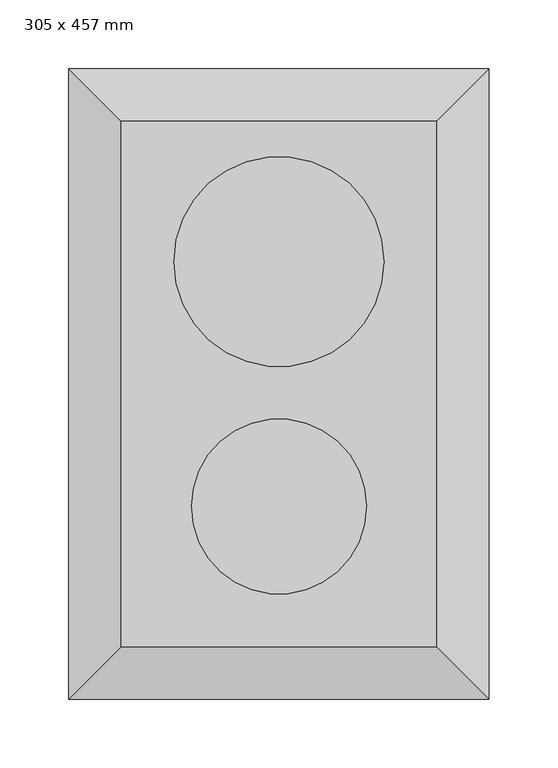
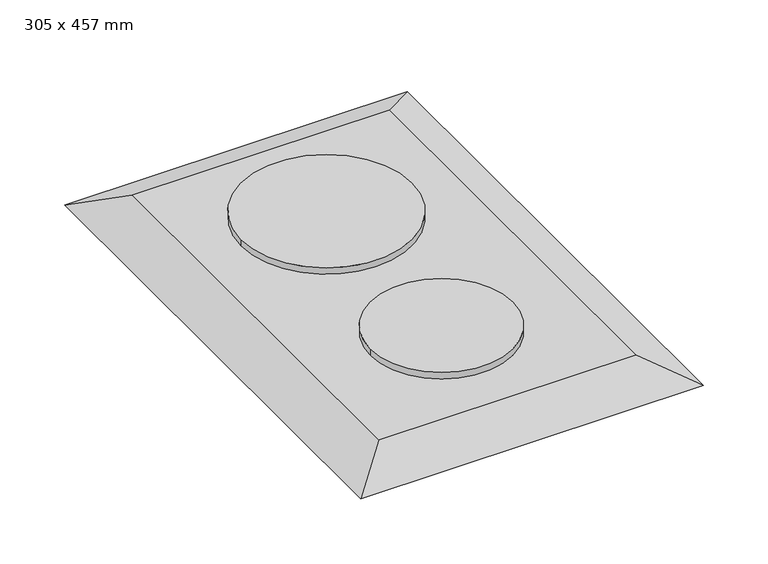
"""IFC4 building model written with IfcOpenShell, lengths in millimetres: proxy geometry, Cocina encimera - 2 fuegos : 305 x 457 mm."""

from ifc_helpers import new_model, si_unit, point, frame, frame_2d, origin, place, context, project, spatial, circle_curve, trimmed, segment, composite_curve, outline, extrude, faceted_brep, source, transform, mapped, element, save


def proxy_305_x_457_mm_75991893(model_context):
    return source(origin(), model_context, "Body", "SolidModel", [
        faceted_brep([(190.6, 220.6247956, 919.05), (-38.2, 220.6247956, 919.05), (-38.2, -160.1752044, 919.05), (190.6, -160.1752044, 919.05), (228.7, 258.7247956, 900.0), (228.7, -198.2752044, 900.0), (-76.3, -198.2752044, 900.0), (-76.3, 258.7247956, 900.0)], [[[0, 1, 2, 3]], [[4, 5, 6, 7]], [[4, 7, 1, 0]], [[7, 6, 2, 1]], [[6, 5, 3, 2]], [[5, 4, 0, 3]]]),
        extrude(outline(composite_curve([segment(trimmed(circle_curve(frame_2d((76.2, 119.0247956)), 76.2), [point((152.4, 119.0247956))], [point((0.0, 119.0247956))], False, "CARTESIAN"), True, "CONTINUOUS"), segment(trimmed(circle_curve(frame_2d((76.2, 119.0247956)), 76.2), [point((0.0, 119.0247956))], [point((152.4, 119.0247956))], False, "CARTESIAN"), True, "CONTINUOUS")], self_intersect=False)), frame((0.0, 0.0, 919.05), z_axis=(0.0, 0.0, 1.0), x_axis=(1.0, 0.0, 0.0)), (0.0, 0.0, 1.0), 6.35),
        extrude(outline(composite_curve([segment(trimmed(circle_curve(frame_2d((76.2, -58.5752044)), 63.5), [point((139.7, -58.5752044))], [point((12.7, -58.5752044))], False, "CARTESIAN"), True, "CONTINUOUS"), segment(trimmed(circle_curve(frame_2d((76.2, -58.5752044)), 63.5), [point((12.7, -58.5752044))], [point((139.7, -58.5752044))], False, "CARTESIAN"), True, "CONTINUOUS")], self_intersect=False)), frame((0.0, 0.0, 919.05), z_axis=(0.0, 0.0, 1.0), x_axis=(1.0, 0.0, 0.0)), (0.0, 0.0, 1.0), 6.35),
    ])


if __name__ == "__main__":
    model = new_model("IFC4")
    model_context = context("Model", 3, world=origin())
    ifc_project = project(units=[si_unit("LENGTHUNIT", "METRE", prefix="MILLI")], contexts=[model_context])
    site = spatial("IfcSite", under=ifc_project)
    building = spatial("IfcBuilding", under=site)
    placement = place(None, origin())
    proxy_305_x_457_mm_shape = proxy_305_x_457_mm_75991893(model_context)
    element("IfcBuildingElementProxy", 1, Name="Cocina encimera - 2 fuegos : 305 x 457 mm", ObjectType="Cocina encimera - 2 fuegos : 305 x 457 mm", at=placement, inside=building, context=model_context, shape_type="MappedRepresentation", body=[
        mapped(proxy_305_x_457_mm_shape, transform((0.0, 0.0, 0.0), x_axis=(1.0, 0.0, 0.0), y_axis=(0.0, 1.0, 0.0), z_axis=(0.0, 0.0, 1.0))),
    ])
    save(model, "model.ifc")

# Revit data of these elements
# Type "Cocina encimera - 2 fuegos : 305 x 457 mm"
#   Altura de encimera = 0.90 m
#   Profundidad = 0.457 m
#   Anchura = 0.305 m
#   Máscara [instance default] = yes
#   Quemador = Metal - Cromo
#   Cocina encimera = Metal - Acero, Pulido
#   Default Elevation = 0
# Element 1 (IfcBuildingElementProxy, "Cocina encimera - 2 fuegos : 305 x 457 mm")
#   Materials on its faces: "Metal - Acero, Pulido", "Metal - Cromo"
# Materials
#   "Metal - Cromo": class "Metal", colour RGB 17 17 17, transparency 0
#   "Metal - Acero, Pulido": class "Metal", colour RGB 57 57 57, transparency 0
